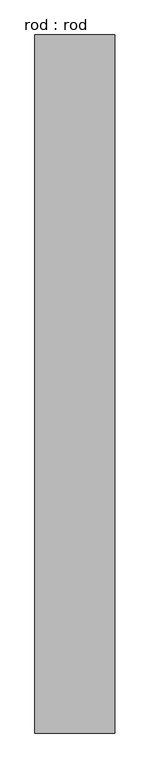
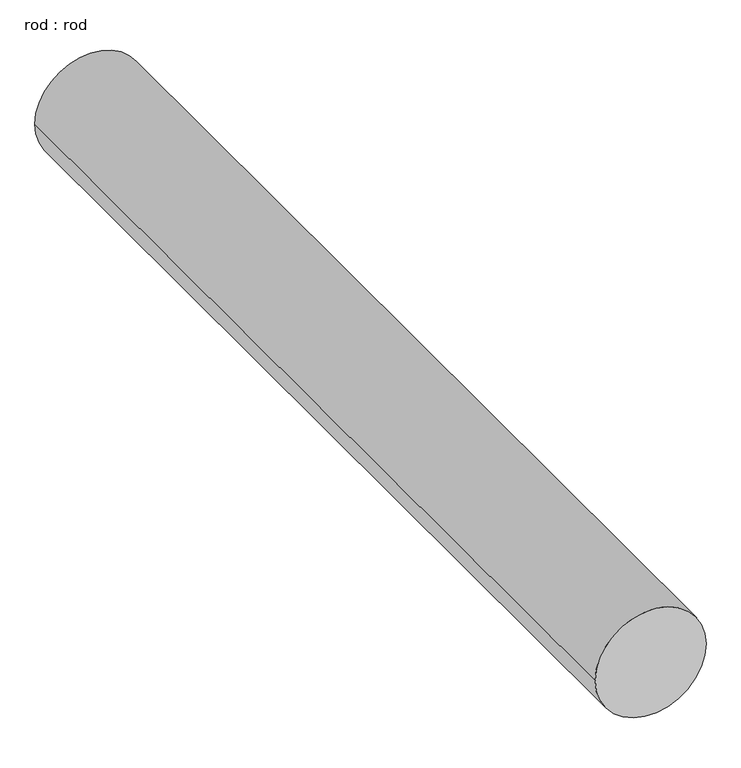
"""IFC4 building model written with IfcOpenShell, lengths in millimetres: proxy geometry, rod : rod."""

from ifc_helpers import new_model, si_unit, point, frame, frame_2d, origin, place, context, project, spatial, circle_curve, trimmed, segment, composite_curve, outline, extrude, source, transform, mapped, element, save


def rod_rod_e1fd1b45(model_context):
    return source(origin(), model_context, "Body", "SweptSolid", [
        extrude(outline(composite_curve([segment(trimmed(circle_curve(frame_2d((0.0108462, 0.0)), 200.0), [point((0.0108462, 200.0))], [point((0.0108462, -200.0))], False, "CARTESIAN"), True, "CONTINUOUS"), segment(trimmed(circle_curve(frame_2d((0.0108462, 0.0)), 200.0), [point((0.0108462, -200.0))], [point((0.0108462, 200.0))], False, "CARTESIAN"), True, "CONTINUOUS")], self_intersect=False)), frame((0.0, 2340.9429011, 0.0), z_axis=(0.0, 1.0, 0.0), x_axis=(0.0, 0.0, 1.0)), (0.0, 0.0, 1.0), 3503.5714286),
    ])


if __name__ == "__main__":
    model = new_model("IFC4")
    model_context = context("Model", 3, world=origin())
    ifc_project = project(units=[si_unit("LENGTHUNIT", "METRE", prefix="MILLI")], contexts=[model_context])
    site = spatial("IfcSite", under=ifc_project)
    building = spatial("IfcBuilding", under=site)
    placement = place(None, origin())
    rod_rod_shape = rod_rod_e1fd1b45(model_context)
    element("IfcBuildingElementProxy", 1, Name="rod : rod", ObjectType="rod : rod", at=placement, inside=building, context=model_context, shape_type="MappedRepresentation", body=[
        mapped(rod_rod_shape, transform((0.0, 0.0, 0.0), x_axis=(1.0, 0.0, 0.0), y_axis=(0.0, 1.0, 0.0), z_axis=(0.0, 0.0, 1.0))),
    ])
    save(model, "model.ifc")

# Revit data of these elements
# Type "rod : rod"
#   Default Elevation = 0
